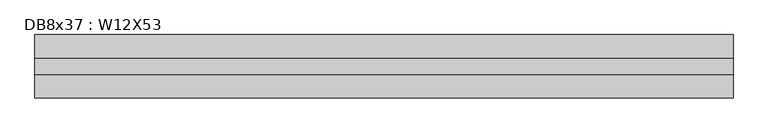
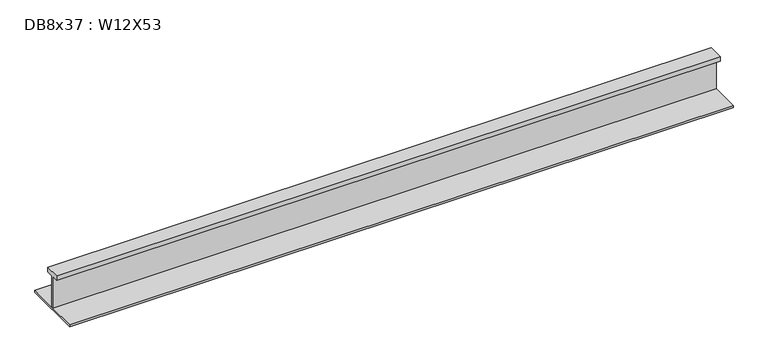
"""IFC4 building model written with IfcOpenShell, lengths in millimetres: beam geometry, DB8x37 : W12X53."""

from ifc_helpers import new_model, si_unit, frame, origin, place, context, project, spatial, polyline, outline, extrude, source, transform, mapped, element, save


def db8x37_w12x53_6089e1ea(model_context):
    return source(origin(), model_context, "Body", "SweptSolid", [
        extrude(outline(polyline([(38.1, 145.415), (38.1, 120.015), (2.921, 120.015), (2.921, -48.4505), (152.4, -48.4505), (152.4, -58.1025), (-152.4, -58.1025), (-152.4, -48.4505), (-2.921, -48.4505), (-2.921, 120.015), (-38.1, 120.015), (-38.1, 145.415), (38.1, 145.415)])), frame((-1649.73, 0.0, 0.0), z_axis=(1.0, 0.0, 0.0), x_axis=(0.0, 1.0, 0.0)), (0.0, 0.0, 1.0), 3352.038),
    ])


if __name__ == "__main__":
    model = new_model("IFC4")
    model_context = context("Model", 3, world=origin())
    ifc_project = project(units=[si_unit("LENGTHUNIT", "METRE", prefix="MILLI")], contexts=[model_context])
    site = spatial("IfcSite", under=ifc_project)
    building = spatial("IfcBuilding", under=site)
    placement = place(None, origin())
    db8x37_w12x53_shape = db8x37_w12x53_6089e1ea(model_context)
    element("IfcBeam", 1, ObjectType="DB8x37 : W12X53", at=placement, inside=building, context=model_context, shape_type="MappedRepresentation", body=[
        mapped(db8x37_w12x53_shape, transform((0.0, 0.0, 0.0), x_axis=(1.0, 0.0, 0.0), y_axis=(0.0, 1.0, 0.0), z_axis=(0.0, 0.0, 1.0))),
    ])
    save(model, "model.ifc")

# Revit data of these elements
# Type "DB8x37 : W12X53"
#   Assembly Code = "B10"
#   W = 53
#   Length [instance default] = 5' - 0"
#   bf = 0' - 10"
#   d = 1' - 0.1"
#   k = 0' - 1 3/8"
#   k2 = 0' - 0.8"
#   tf = 0' - 0.575"
#   tw = 0' - 0.345"
#   A = 0.108333 SF
#   Structural Material [instance default] = Steel ASTM A992
# Element 1 (IfcBeam, "DB8x37 : W12X53")
#   Materials on its faces: "Steel ASTM A992"
# Materials
#   "Steel ASTM A992": class "Metal", colour RGB 199 199 199, transparency 0, Description = "Structural steel 50ksi", Cost = 0
